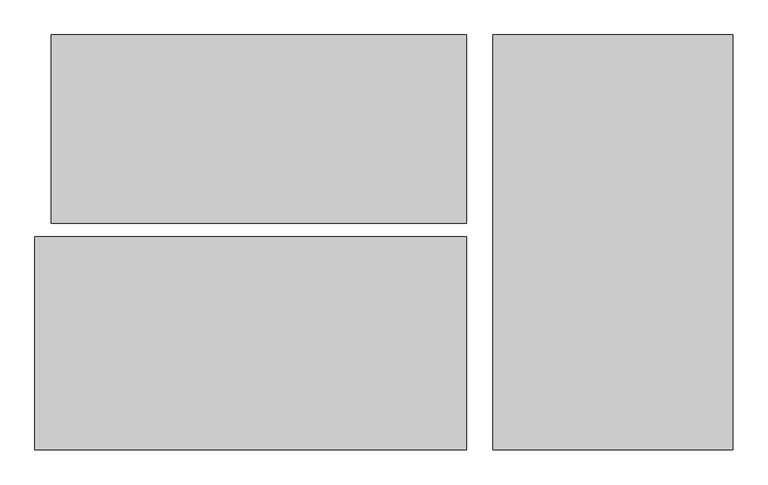
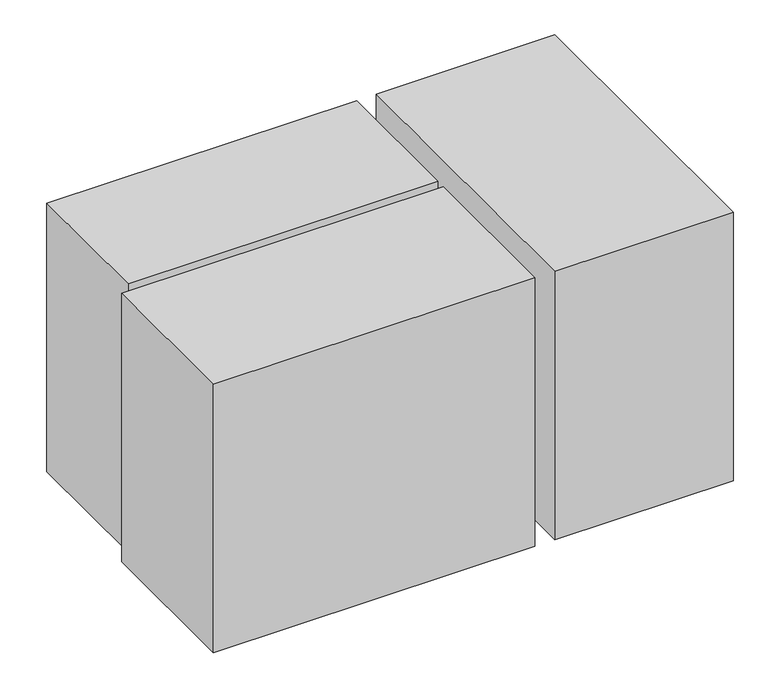
"""IFC4 building model written with IfcOpenShell, lengths in millimetres: proxy geometry, 0_3d_modell."""

from ifc_helpers import new_model, si_unit, origin, origin_with_axes, place, context, project, spatial, polyline, outline, extrude, source, transform, mapped, element, save


def generic_models_359e7ffc(model_context):
    return source(origin(), model_context, "Body", "SweptSolid", [
        extrude(outline(polyline([(3461.9364642, 0.0), (3461.9364642, 3133.4), (5272.0, 3133.4), (5272.0, 0.0), (3461.9364642, 0.0)])), origin_with_axes(), (0.0, 0.0, 1.0), 2880.0),
        extrude(outline(polyline([(3261.9364642, 3133.4), (3261.9364642, 1709.3795824), (122.0, 1709.3795824), (122.0, 3133.4), (3261.9364642, 3133.4)])), origin_with_axes(), (0.0, 0.0, 1.0), 2880.0),
        extrude(outline(polyline([(0.0, 0.0), (0.0, 1609.3795824), (3261.9364642, 1609.3795824), (3261.9364642, 0.0), (0.0, 0.0)])), origin_with_axes(), (0.0, 0.0, 1.0), 2880.0),
    ])


if __name__ == "__main__":
    model = new_model("IFC4")
    model_context = context("Model", 3, world=origin())
    ifc_project = project(units=[si_unit("LENGTHUNIT", "METRE", prefix="MILLI")], contexts=[model_context])
    site = spatial("IfcSite", under=ifc_project)
    building = spatial("IfcBuilding", under=site)
    placement = place(None, origin())
    generic_models_shape = generic_models_359e7ffc(model_context)
    element("IfcBuildingElementProxy", 1, Name="0_3d_modell", ObjectType="0_3d_modell", at=placement, inside=building, context=model_context, shape_type="MappedRepresentation", body=[
        mapped(generic_models_shape, transform((0.0, 0.0, 0.0), x_axis=(1.0, 0.0, 0.0), y_axis=(0.0, 1.0, 0.0), z_axis=(0.0, 0.0, 1.0))),
    ])
    save(model, "model.ifc")

# Revit data of these elements
# Element 1 (IfcBuildingElementProxy, "0_3d_modell")
#   Materials on its faces: "*1"
# Materials
#   "*1": class "Unassigned", colour RGB 175 175 175, transparency 0
